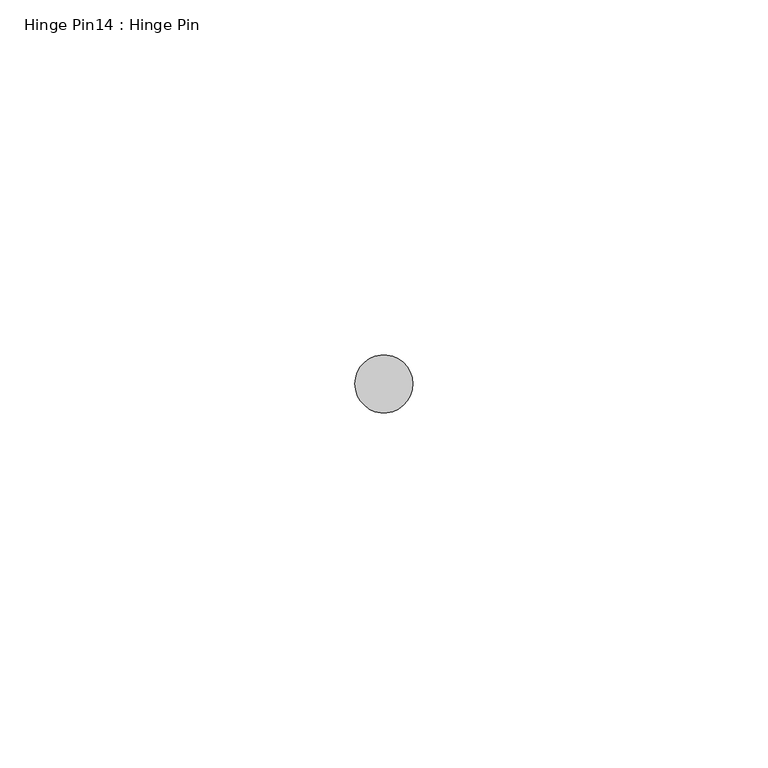
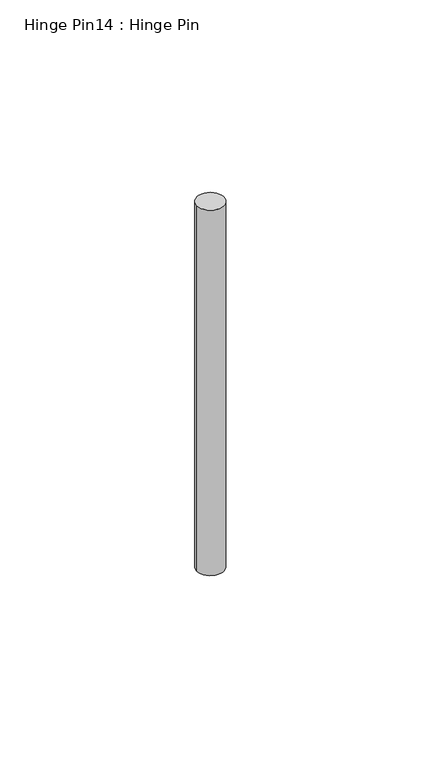
"""IFC4 building model written with IfcOpenShell, lengths in millimetres: proxy geometry, Hinge Pin14 : Hinge Pin."""

import ifcopenshell
import ifcopenshell.guid

model = None  # the IFC model being written
_history = None  # IfcOwnerHistory: only IFC2X3 demands one
_inside = {}  # id of a spatial element -> (the spatial element, [elements in it])
_under = {}  # id of a project, library or spatial element -> (it, [spatial elements below it])
_declared = {}  # id of a project -> (the project, [libraries it declares])
_typed = {}  # id of a type object -> (the type object, [elements of that type])
_made_of = {}  # id of a material, layer set ... -> (it, [elements and type objects made of it])


def new_model(schema):
    """Start an empty IFC model of exactly this schema.

    Asked for "IFC4X3", IfcOpenShell would pick the latest addendum, in which some entities
    have other attributes; the version numbers below select the first issue.
    IFC2X3 requires an IfcOwnerHistory on every rooted entity: one is made here for all.
    """
    global model, _history
    if schema == "IFC4X3":
        model = ifcopenshell.file(schema_version=(4, 3, 0, 0))
    else:
        model = ifcopenshell.file(schema=schema)
    _inside.clear()
    _under.clear()
    _declared.clear()
    _typed.clear()
    _made_of.clear()
    _history = None
    if model.schema == "IFC2X3":
        org = make("IfcOrganization", Name="unknown")
        user = make(
            "IfcPersonAndOrganization",
            ThePerson=make("IfcPerson", FamilyName="unknown"),
            TheOrganization=org,
        )
        app = make(
            "IfcApplication",
            ApplicationDeveloper=org,
            Version="unknown",
            ApplicationFullName="unknown",
            ApplicationIdentifier="unknown",
        )
        _history = make(
            "IfcOwnerHistory",
            OwningUser=user,
            OwningApplication=app,
            ChangeAction="ADDED",
            CreationDate=0,
        )
    return model


def make(cls, **values):
    """One entity of the class cls with the attributes given. An attribute that is None is left unset."""
    return model.create_entity(
        cls, **{name: value for name, value in values.items() if value is not None}
    )


def rooted(cls, **values):
    """An entity with a GlobalId (a new one), such as an element, a storey or a relation."""
    return make(cls, GlobalId=ifcopenshell.guid.new(), OwnerHistory=_history, **values)


def si_unit(unit_type, name, prefix=None):
    """IfcSIUnit, for example si_unit("LENGTHUNIT", "METRE", prefix="MILLI")."""
    return make("IfcSIUnit", UnitType=unit_type, Prefix=prefix, Name=name)


def assignment(units):
    """IfcUnitAssignment: the units of a project."""
    return None if units is None else make("IfcUnitAssignment", Units=units)


def point(xyz):
    """IfcCartesianPoint."""
    return None if xyz is None else make("IfcCartesianPoint", Coordinates=xyz)


def direction(xyz):
    """IfcDirection."""
    return None if xyz is None else make("IfcDirection", DirectionRatios=xyz)


def frame(location, z_axis=None, x_axis=None):
    """IfcAxis2Placement3D, a coordinate frame: its origin and axes. An axis left out is left unset."""
    return make(
        "IfcAxis2Placement3D",
        Location=point(location),
        Axis=direction(z_axis),
        RefDirection=direction(x_axis),
    )


def frame_2d(location, x_axis=None):
    """IfcAxis2Placement2D, a coordinate frame in the plane: its origin and x axis."""
    return make(
        "IfcAxis2Placement2D", Location=point(location), RefDirection=direction(x_axis)
    )


def origin():
    """The frame at (0, 0, 0) with its axes left unset."""
    return frame((0.0, 0.0, 0.0))


def place(relative_to, where):
    """IfcLocalPlacement: puts the frame where relative to a parent placement (None: the world)."""
    return make(
        "IfcLocalPlacement", PlacementRelTo=relative_to, RelativePlacement=where
    )


def context(
    kind, dimensions, precision=None, world=None, true_north=None, identifier=None
):
    """IfcGeometricRepresentationContext, for example the 3D "Model" context."""
    return make(
        "IfcGeometricRepresentationContext",
        ContextIdentifier=identifier,
        ContextType=kind,
        CoordinateSpaceDimension=dimensions,
        Precision=precision,
        WorldCoordinateSystem=world,
        TrueNorth=true_north,
    )


def project(units=None, contexts=None):
    """IfcProject with its units and contexts."""
    return rooted(
        "IfcProject",
        Name="project",
        RepresentationContexts=contexts,
        UnitsInContext=assignment(units),
    )


def spatial(cls, under=None, at=None, **own):
    """A site, building, storey or space (cls), placed at a placement, below another one or the project."""
    s = rooted(cls, ObjectPlacement=at, **own)
    if under is not None:
        _under.setdefault(under.id(), (under, []))[1].append(s)
    return s


def circle_curve(where, radius):
    """IfcCircle in the frame where."""
    return make("IfcCircle", Position=where, Radius=radius)


def trimmed(basis, trim1, trim2, sense, master):
    """IfcTrimmedCurve: the piece of a basis curve between two trims."""
    return make(
        "IfcTrimmedCurve",
        BasisCurve=basis,
        Trim1=trim1,
        Trim2=trim2,
        SenseAgreement=sense,
        MasterRepresentation=master,
    )


def segment(curve, same_sense, transition):
    """IfcCompositeCurveSegment."""
    return make(
        "IfcCompositeCurveSegment",
        Transition=transition,
        SameSense=same_sense,
        ParentCurve=curve,
    )


def composite_curve(segments, self_intersect=None):
    """IfcCompositeCurve: segments joined end to end."""
    return make("IfcCompositeCurve", Segments=segments, SelfIntersect=self_intersect)


def outline(outer, holes=None, kind="AREA"):
    """IfcArbitraryClosedProfileDef: a profile drawn as a closed curve; with holes, ...WithVoids."""
    if holes is None:
        return make("IfcArbitraryClosedProfileDef", ProfileType=kind, OuterCurve=outer)
    return make(
        "IfcArbitraryProfileDefWithVoids",
        ProfileType=kind,
        OuterCurve=outer,
        InnerCurves=holes,
    )


def extrude(swept, where, along, depth):
    """IfcExtrudedAreaSolid: the profile swept, set in the frame where, extruded along a direction by depth."""
    return make(
        "IfcExtrudedAreaSolid",
        SweptArea=swept,
        Position=where,
        ExtrudedDirection=direction(along),
        Depth=depth,
    )


def shape(context_of_items, identifier, shape_type, items):
    """IfcShapeRepresentation: the items that make up one representation, for example the "Body"."""
    return make(
        "IfcShapeRepresentation",
        ContextOfItems=context_of_items,
        RepresentationIdentifier=identifier,
        RepresentationType=shape_type,
        Items=items,
    )


def source(mapping_origin, context_of_items, identifier, shape_type, items):
    """IfcRepresentationMap: a shape defined once, which mapped items show again and again."""
    return make(
        "IfcRepresentationMap",
        MappingOrigin=mapping_origin,
        MappedRepresentation=shape(context_of_items, identifier, shape_type, items),
    )


def transform(
    local_origin,
    x_axis=None,
    y_axis=None,
    z_axis=None,
    scale=None,
    scale2=None,
    scale3=None,
    uniform=True,
):
    """IfcCartesianTransformationOperator3D, or its non-uniform kind. x_axis, y_axis, z_axis: its Axis1, 2, 3."""
    if uniform:
        return make(
            "IfcCartesianTransformationOperator3D",
            Axis1=direction(x_axis),
            Axis2=direction(y_axis),
            LocalOrigin=point(local_origin),
            Scale=scale,
            Axis3=direction(z_axis),
        )
    return make(
        "IfcCartesianTransformationOperator3DnonUniform",
        Axis1=direction(x_axis),
        Axis2=direction(y_axis),
        LocalOrigin=point(local_origin),
        Scale=scale,
        Axis3=direction(z_axis),
        Scale2=scale2,
        Scale3=scale3,
    )


def mapped(mapping_source, mapping_target):
    """IfcMappedItem: shows the shape of a source again, moved by a transform."""
    return make(
        "IfcMappedItem", MappingSource=mapping_source, MappingTarget=mapping_target
    )


def made_of(thing, what):
    """Note that an element or type object is made of a material, layer set ...; save() writes the relation."""
    if what is not None:
        _made_of.setdefault(what.id(), (what, []))[1].append(thing)
    return thing


def element(
    cls,
    number,
    at=None,
    inside=None,
    cuts=None,
    type_object=None,
    material=None,
    context=None,
    identifier="Body",
    shape_type=None,
    held_by="IfcProductDefinitionShape",
    body=None,
    shapes=None,
    **own,
):
    """One element of the class cls, such as IfcWall. Its Tag is "e" and its number.

    at: its placement. inside: the storey or other place that contains it. cuts: it is an
    opening in that element (IfcRelVoidsElement). A single representation is given by context,
    identifier, shape_type and body (its items); several are given by shapes. held_by: the class
    of the entity that holds the representations. save() writes the other relations.
    """
    e = rooted(cls, Tag="e%d" % number, ObjectPlacement=at, **own)
    if body is not None:
        shapes = [shape(context, identifier, shape_type, body)]
    if shapes is not None:
        e.Representation = make(held_by, Representations=shapes)
    if inside is not None:
        _inside.setdefault(inside.id(), (inside, []))[1].append(e)
    if cuts is not None:
        rooted(
            "IfcRelVoidsElement", RelatingBuildingElement=cuts, RelatedOpeningElement=e
        )
    if type_object is not None:
        _typed.setdefault(type_object.id(), (type_object, []))[1].append(e)
    return made_of(e, material)


def aggregate(whole, parts):
    """IfcRelAggregates: a whole, such as a stair, and the parts it consists of."""
    return rooted("IfcRelAggregates", RelatingObject=whole, RelatedObjects=parts)


def save(model, path):
    """Write the relations noted so far, then the file.

    IfcRelAggregates (storeys below a building ...), IfcRelContainedInSpatialStructure (elements
    in a storey), IfcRelDefinesByType, IfcRelAssociatesMaterial and IfcRelDeclares: one each for
    every whole, place, type object, material and project.
    """
    for whole, parts in _under.values():
        aggregate(whole, parts)
    for where, things in _inside.values():
        rooted(
            "IfcRelContainedInSpatialStructure",
            RelatedElements=things,
            RelatingStructure=where,
        )
    for kind, things in _typed.values():
        rooted("IfcRelDefinesByType", RelatedObjects=things, RelatingType=kind)
    for what, things in _made_of.values():
        rooted("IfcRelAssociatesMaterial", RelatedObjects=things, RelatingMaterial=what)
    for by, libraries in _declared.values():
        rooted("IfcRelDeclares", RelatingContext=by, RelatedDefinitions=libraries)
    model.write(path)


def hinge_pin14_hinge_pin_c21d8c14(model_context):
    return source(origin(), model_context, "Body", "SweptSolid", [
        extrude(outline(composite_curve([segment(trimmed(circle_curve(frame_2d((587319.1320739, -531776.6049841)), 4.0894), [point((587315.0426739, -531776.6049841))], [point((587323.2214739, -531776.6049841))], False, "CARTESIAN"), True, "CONTINUOUS"), segment(trimmed(circle_curve(frame_2d((587319.1320739, -531776.6049841)), 4.0894), [point((587323.2214739, -531776.6049841))], [point((587315.0426739, -531776.6049841))], False, "CARTESIAN"), True, "CONTINUOUS")], self_intersect=False)), frame((0.0, 0.0, 1128.5140625), z_axis=(0.0, 0.0, 1.0), x_axis=(1.0, 0.0, 0.0)), (0.0, 0.0, 1.0), 117.871875),
    ])


if __name__ == "__main__":
    model = new_model("IFC4")
    model_context = context("Model", 3, world=origin())
    ifc_project = project(units=[si_unit("LENGTHUNIT", "METRE", prefix="MILLI")], contexts=[model_context])
    site = spatial("IfcSite", under=ifc_project)
    building = spatial("IfcBuilding", under=site)
    placement = place(None, origin())
    hinge_pin14_hinge_pin_shape = hinge_pin14_hinge_pin_c21d8c14(model_context)
    element("IfcBuildingElementProxy", 1, Name="Hinge Pin14 : Hinge Pin", ObjectType="Hinge Pin14 : Hinge Pin", at=placement, inside=building, context=model_context, shape_type="MappedRepresentation", body=[
        mapped(hinge_pin14_hinge_pin_shape, transform((0.0, 0.0, 0.0), x_axis=(1.0, 0.0, 0.0), y_axis=(0.0, 1.0, 0.0), z_axis=(0.0, 0.0, 1.0))),
    ])
    save(model, "model.ifc")

# Revit data of these elements
# Element 1 (IfcBuildingElementProxy, "Hinge Pin14 : Hinge Pin")
#   Materials on its faces: "6\"X6\" WELD-ON STL BUTT HINGE"
# Materials
#   "6\"X6\" WELD-ON STL BUTT HINGE": class "Metal", colour RGB 189 187 185, transparency 0, Description = "Carbon steel", Cost = 0
